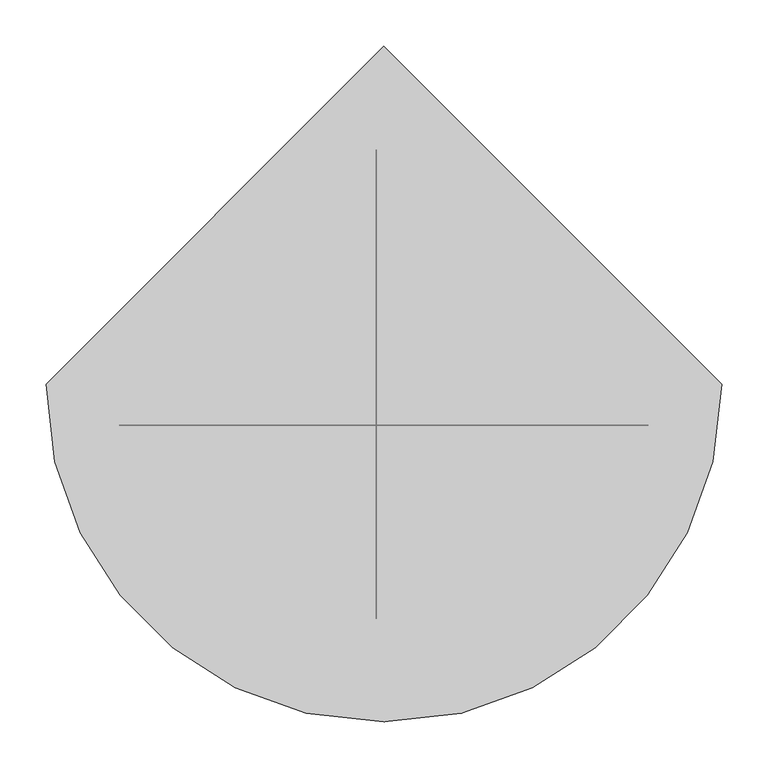
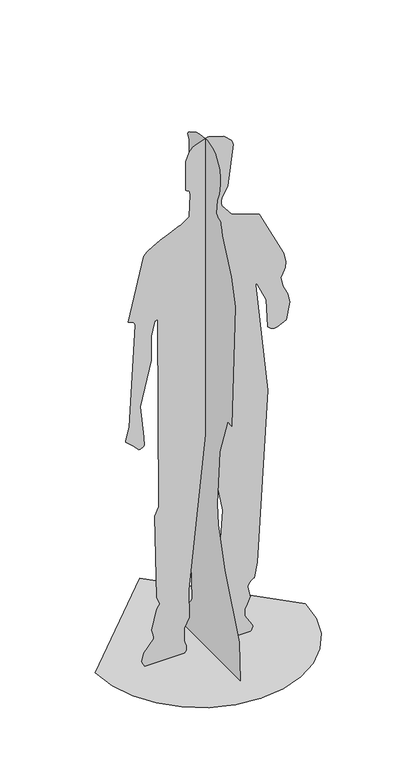
"""IFC4 building model written with IfcOpenShell, lengths in millimetres: proxy geometry, adam 24238 : adam 24238."""

from ifc_helpers import new_model, si_unit, origin, place, context, project, spatial, triangles, source, transform, mapped, element, save


def entourage_3dd67646(model_context):
    return source(origin(), model_context, "Body", "Tessellation", [
        triangles([(-366.6435362, 0.0, 0.0002608), (-356.9509229, -84.0106697, 0.0002608), (-329.3462125, -161.1608025, 0.0002608), (-286.0392629, -229.2406041, 0.0002608), (-229.2406041, -286.0392629, 0.0002608), (-161.1608025, -329.3462125, 0.0002608), (-84.0104153, -356.9509229, 0.0002608), (1.6e-05, -366.6435362, 0.0002608), (84.0106697, -356.9509229, 0.0002608), (161.1608025, -329.3462125, 0.0002608), (229.2406041, -286.0392629, 0.0002608), (286.0392629, -229.2406041, 0.0002608), (329.3462125, -161.1608025, 0.0002608), (356.9509229, -84.0104153, 0.0002608), (366.6435362, 3.21e-05, 0.0002608), (-4.81e-05, 366.6435362, 0.0002608), (-1.944876, -44.4273482, 1879.2018654), (3.9408568, -44.4273482, 1879.5980621), (56.9254043, -44.4273482, 1862.3235352), (60.0092186, -44.4273482, 1860.464201), (82.4127567, -44.4273482, 1839.6871262), (84.7807989, -44.4273482, 1835.3868073), (86.2341804, -44.4273482, 1831.4396645), (87.2151253, -44.4273482, 1827.7541336), (88.1663572, -44.4273482, 1824.2387959), (89.5305907, -44.4273482, 1820.8022324), (69.8819309, -44.4273482, 1675.5804279), (49.8977401, -44.4273482, 1635.9869144), (47.4702674, -44.4273482, 1627.3306114), (46.8911467, -44.4273482, 1618.12565), (48.8728526, -44.4273482, 1608.5092312), (84.8181331, -44.4273482, 1564.6994053), (180.6730562, -44.4273482, 1530.7014805), (265.4856119, -44.4273482, 1357.9816452), (273.9031577, -44.4273482, 1321.9899467), (272.1200725, -44.4273482, 1302.5614815), (259.6918704, -44.4273482, 1276.1125145), (255.5592919, -44.4273482, 1271.5937496), (262.6230323, -44.4273482, 1237.7838947), (280.4588985, -44.4273482, 1201.9495995), (287.0120778, -44.4273482, 1169.7501114), (275.2163406, -44.4273482, 1107.5938036), (243.3053342, -44.4273482, 1092.5062071), (232.2253601, -44.4273482, 1091.4673897), (221.1288717, -44.4273482, 1094.7134851), (210.6275142, -44.4273482, 1103.8498461), (204.6366735, -44.4273482, 1205.693557), (173.7175396, -44.4273482, 1274.9364235), (170.1887216, -44.4273482, 1279.8310375), (168.2918534, -44.4273482, 1273.0009312), (210.6275142, -44.4273482, 870.2031338), (173.1843963, -44.4273482, 247.1475961), (162.7002979, -44.4273482, 193.2292847), (158.5405409, -44.4273482, 191.6712584), (154.4254941, -44.4273482, 189.1513178), (150.5182108, -44.4273482, 185.873193), (143.9807646, -44.4273482, 177.8600194), (140.2342727, -44.4273482, 169.2656857), (139.8659722, -44.4273482, 165.4886996), (148.7468164, -44.4273482, 128.2548804), (146.2251135, -44.4273482, 121.3384694), (135.4476463, -44.4273482, 98.5313222), (129.7501834, -44.4273482, 91.3837752), (130.189855, -44.4273482, 64.5309176), (156.6515392, -44.4273482, 21.8279259), (157.9146888, -44.4273482, 16.6136911), (151.2215381, -44.4273482, 0.0003058), (84.0693416, -44.4273482, 0.0003058), (74.1432851, -44.4273482, 0.0003058), (38.7179401, -44.4273482, 0.0003058), (33.3654053, -44.4273482, 7.4764826), (29.9579983, -44.4273482, 15.6459779), (30.9000852, -44.4273482, 79.4020938), (5.8130383, -44.4273482, 108.6077512), (16.2900951, -44.4273482, 154.9116381), (26.428926, -44.4273482, 174.7358278), (31.8360723, -44.4273482, 178.7200504), (53.3658514, -44.4273482, 480.7935817), (-0.5087539, -44.4273482, 768.3289015), (-4.8489568, -44.4273482, 778.4024872), (-8.1273059, -44.4273482, 782.5858801), (-66.7455444, -44.4273482, 230.3825947), (-64.9545927, -44.4273482, 127.3293101), (-82.1785686, -44.4273482, 92.8816126), (-82.0467452, -44.4273482, 50.1072885), (-79.3850799, -44.4273482, 38.292748), (-77.114579, -44.4273482, 31.7072965), (-75.2644421, -44.4273482, 24.8938543), (-74.7376438, -44.4273482, 21.6405237), (-73.9411035, -44.4273482, 8.9179564), (-82.2286019, -44.4273482, 0.0003058), (-167.3571176, -44.4273482, 0.0003058), (-195.4322207, -44.4273482, 0.0003058), (-220.693524, -44.4273482, 0.0003058), (-229.0292798, -44.4273482, 16.7492252), (-230.8413058, -44.4273482, 20.814543), (-222.9200778, -44.4273482, 48.8121459), (-189.2661364, -44.4273482, 91.3837752), (-188.5071711, -44.4273482, 95.7134528), (-189.5673716, -44.4273482, 106.4002369), (-195.2572133, -44.4273482, 124.3338897), (-177.4482894, -44.4273482, 196.2374042), (-171.6923907, -44.4273482, 207.2632755), (-166.6131586, -44.4273482, 211.9511071), (-178.7820379, -44.4273482, 241.1567554), (-184.9603309, -44.4273482, 542.7618922), (-171.2933599, -44.4273482, 573.6533206), (-173.5918024, -44.4273482, 1268.7160183), (-176.5392242, -44.4273482, 1266.3157288), (-180.7269047, -44.4273482, 1264.2963753), (-184.1635227, -44.4273482, 1262.873933), (-196.7547963, -44.4273482, 1211.6854151), (-197.4888539, -44.4273482, 1123.6948557), (-235.7404617, -44.4273482, 964.4218014), (-222.7747923, -44.4273482, 847.8637997), (-222.2916823, -44.4273482, 817.8105469), (-224.3125073, -44.4273482, 813.6982979), (-236.1842028, -44.4273482, 807.6734476), (-240.250488, -44.4273482, 807.7775837), (-258.0789783, -44.4273482, 826.659934), (-286.6183881, -44.4273482, 852.2301029), (-287.0120778, -44.4273482, 857.7164686), (-274.6372154, -44.4273482, 903.1544655), (-252.8453043, -44.4273482, 1272.1043289), (-256.6642027, -44.4273482, 1280.580265), (-259.0238515, -44.4273482, 1283.9636341), (-262.7017702, -44.4273482, 1287.1919254), (-277.6318727, -44.4273482, 1292.5639812), (-223.7140882, -44.4273482, 1517.22178), (-211.4377663, -44.4273482, 1529.2765675), (-191.0382847, -44.4273482, 1542.4388454), (-166.1168408, -44.4273482, 1555.6290287), (-140.2749134, -44.4273482, 1567.7650612), (-117.1134366, -44.4273482, 1577.7727352), (-100.2331261, -44.4273482, 1584.5672333), (-93.235688, -44.4273482, 1587.0715862), (-64.9545927, -44.4273482, 1608.5092312), (-60.4615893, -44.4273482, 1689.3852539), (-64.9545927, -44.4273482, 1704.3637001), (-72.9002105, -44.4273482, 1706.6725708), (-76.9365194, -44.4273482, 1710.3554855), (-76.9365194, -44.4273482, 1815.1964699), (-63.7389465, -44.4273482, 1845.7348675), (-52.4684725, -44.4273482, 1859.6082939), (-45.3999133, -44.4273482, 1864.0863636), (-8.0256042, -11.9576731, 1872.7679558), (-8.0256042, 11.9818279, 1866.0065952), (-8.0256042, 15.3371645, 1863.8221355), (-8.0256042, 22.6286333, 1860.1111702), (-8.0256042, 52.1745951, 1843.9237862), (-8.0256042, 59.2657593, 1838.2062572), (-8.0256042, 62.1903128, 1832.0620102), (-8.0256042, 53.0188886, 1813.7892883), (-8.0256042, 52.9246538, 1765.8900318), (-8.0256042, 44.5975276, 1745.3719528), (-8.0256042, 43.1614143, 1739.042252), (-8.0256042, 42.5904236, 1733.5252922), (-8.0256042, 43.7575489, 1727.7036999), (-8.0256042, 55.0026293, 1710.038063), (-8.0256042, 56.3198681, 1705.2323971), (-8.0256042, 56.3130144, 1700.5637867), (-8.0256042, 54.9551303, 1697.4193565), (-8.0256042, 51.5324831, 1692.3012096), (-8.0256042, 42.342519, 1638.3515957), (-8.0256042, 37.5670701, 1634.3867214), (-8.0256042, 32.4891075, 1633.1116539), (-8.0256042, 26.9745186, 1632.7509201), (-8.0256042, 10.5312862, 1632.4512291), (-8.0256042, 5.990914, 1631.0491344), (-8.0256042, -10.8585396, 1605.5881886), (-8.0256042, -12.7524636, 1593.756934), (-8.0256042, -14.0942421, 1561.7504574), (-8.0256042, -12.4802009, 1555.913459), (-8.0256042, -0.6249435, 1547.4248783), (-8.0256042, 1.123296, 1487.2675037), (-8.0256042, 62.9045588, 1181.7312841), (-8.0256042, 204.7502021, 1194.7106518), (-8.0256042, 240.9944469, 1187.0627174), (-8.0256042, 245.2555422, 1184.3373024), (-8.0256042, 248.1186306, 1181.6397926), (-8.0256042, 250.7140027, 1178.419059), (-8.0256042, 252.8133113, 1174.7919548), (-8.0256042, 254.190244, 1170.8651596), (-8.0256042, 254.6144186, 1166.7529106), (-8.0256042, 252.0965127, 1160.1615978), (-8.0256042, 209.0618576, 1117.5633259), (-8.0256042, 200.8416653, 1117.1137167), (-8.0256042, 154.1989273, 1133.9615255), (-8.0256042, 137.6038465, 1140.5426645), (-8.0256042, 128.3780742, 1142.4908014), (-8.0256042, 118.7530076, 1142.7423122), (-8.0256042, 91.266931, 1137.6775051), (-8.0256042, 83.8282953, 1135.5007484), (-8.0256042, 77.8819104, 1133.8040497), (-8.0256042, 107.8363502, 921.1249529), (-8.0256042, 77.8819104, 924.1221537), (-8.0256042, 65.8999792, 456.8286927), (-8.0256042, 47.1936582, 374.7740719), (-8.0256042, 36.3199306, 128.765169), (-8.0256042, 38.6638419, 122.1693053), (-8.0256042, 45.3846753, 111.9155889), (-8.0256042, 54.7316111, 99.4668029), (-8.0256042, 64.9538296, 86.2865028), (-8.0256042, 74.3007655, 73.8377259), (-8.0256042, 77.1531849, 69.6548554), (-8.0256042, 85.0581621, 63.3091807), (-8.0256042, 97.368766, 60.2769303), (-8.0256042, 127.5726364, 57.0927906), (-8.0256042, 134.7956331, 56.8740993), (-8.0256042, 155.3528358, 55.5908928), (-8.0256042, 161.7546616, 53.878679), (-8.0256042, 166.2479011, 4.4535808), (-8.0256042, 137.0691771, 0.0002528), (-8.0256042, 128.8367944, 0.0002532), (-8.0256042, 121.8759366, 0.0002535), (-8.0256042, 117.0100635, 0.0002537), (-8.0256042, 48.9467671, 0.0002567), (-8.0256042, 31.4243401, 0.0002575), (-8.0256042, 24.3088155, 0.0002578), (-8.0256042, 0.7015143, 0.0002588), (-8.0256042, -24.0727244, 0.0002599), (-8.0255537, -254.6144186, 0.0), (-8.0255537, -248.6230692, 138.153504), (-8.0256042, -160.756939, 352.2239948), (-8.0256042, -121.7822104, 495.2512384), (-8.0256042, -116.8228656, 570.6561198), (-8.0256042, -131.8002127, 771.3540075), (-8.0256042, -179.7276742, 912.1384375), (-8.0255537, -203.6912733, 909.1437801), (-8.0255537, -226.1570532, 1364.4536339), (-8.0255537, -199.9978759, 1460.4934113), (-8.0256042, -169.3555966, 1535.006741), (-8.0256042, -147.61906, 1580.8308334), (-8.0256042, -142.8377657, 1595.5425808), (-8.0256042, -138.9363323, 1616.7312584), (-8.0256042, -137.2446932, 1621.2904278), (-8.0256042, -133.7301003, 1625.7405922), (-8.0256042, -128.0097736, 1628.0545498), (-8.0256042, -123.0057277, 1629.601403), (-8.0256042, -118.2638024, 1630.7520596), (-8.0256042, -115.801271, 1634.0717697), (-8.0256042, -113.8274453, 1638.5065281), (-8.0256042, -111.5132515, 1642.3217022), (-8.0256042, -117.9460529, 1693.2055149), (-8.0256042, -128.7237653, 1721.4399834), (-8.0256042, -135.6343355, 1760.7313351), (-8.0256042, -135.6241799, 1785.6739986), (-8.0256042, -131.8002127, 1813.7715569), (-8.0256042, -114.0471539, 1843.6088345), (-8.0256042, -105.9849461, 1853.79673), (-8.0256042, -97.1990998, 1861.6657265), (-8.0256042, -86.7393912, 1867.8404949), (-8.0256042, -56.9985558, 1877.6016724)], [[15, 16, 1], [14, 15, 1], [14, 1, 2], [13, 14, 2], [13, 2, 3], [13, 3, 4], [12, 13, 4], [11, 12, 4], [11, 4, 5], [11, 5, 6], [11, 6, 7], [11, 7, 8], [11, 8, 9], [11, 9, 10], [66, 67, 68], [115, 116, 117], [52, 53, 54], [66, 68, 69], [66, 69, 70], [66, 70, 71], [65, 66, 71], [65, 71, 72], [65, 72, 73], [64, 65, 73], [63, 64, 73], [89, 90, 91], [127, 128, 129], [62, 63, 73], [61, 62, 73], [61, 73, 74], [61, 74, 75], [61, 75, 76], [61, 76, 77], [60, 61, 77], [59, 60, 77], [58, 59, 77], [57, 58, 77], [56, 57, 77], [56, 77, 78], [55, 56, 78], [54, 55, 78], [52, 54, 78], [51, 52, 78], [51, 78, 79], [51, 79, 80], [51, 80, 81], [45, 46, 47], [44, 45, 47], [43, 44, 47], [42, 43, 47], [41, 42, 47], [40, 41, 47], [39, 40, 47], [38, 39, 47], [38, 47, 48], [38, 48, 49], [37, 38, 49], [36, 37, 49], [35, 36, 49], [34, 35, 49], [33, 34, 49], [32, 33, 49], [95, 96, 97], [94, 95, 97], [93, 94, 97], [92, 93, 97], [91, 92, 97], [91, 97, 98], [91, 98, 99], [89, 91, 99], [88, 89, 99], [87, 88, 99], [86, 87, 99], [85, 86, 99], [84, 85, 99], [84, 99, 100], [84, 100, 101], [83, 84, 101], [83, 101, 102], [83, 102, 103], [83, 103, 104], [82, 83, 104], [82, 104, 105], [82, 105, 106], [82, 106, 107], [82, 107, 108], [81, 82, 108], [51, 81, 108], [50, 51, 108], [49, 50, 108], [32, 49, 108], [31, 32, 108], [30, 31, 108], [118, 119, 120], [117, 118, 120], [115, 117, 120], [115, 120, 121], [115, 121, 122], [115, 122, 123], [114, 115, 123], [114, 123, 124], [113, 114, 124], [112, 113, 124], [111, 112, 124], [111, 124, 125], [111, 125, 126], [110, 111, 126], [109, 110, 126], [108, 109, 126], [30, 108, 126], [30, 126, 127], [30, 127, 129], [30, 129, 130], [30, 130, 131], [30, 131, 132], [30, 132, 133], [30, 133, 134], [30, 134, 135], [30, 135, 136], [30, 136, 137], [30, 137, 138], [29, 30, 138], [28, 29, 138], [27, 28, 138], [27, 138, 139], [26, 27, 139], [25, 26, 139], [24, 25, 139], [23, 24, 139], [22, 23, 139], [21, 22, 139], [20, 21, 139], [19, 20, 139], [18, 19, 139], [17, 18, 139], [145, 17, 139], [144, 145, 139], [143, 144, 139], [142, 143, 139], [141, 142, 139], [141, 139, 140], [194, 195, 196], [221, 222, 223], [221, 223, 224], [220, 221, 224], [219, 220, 224], [218, 219, 224], [217, 218, 224], [216, 217, 224], [215, 216, 224], [214, 215, 224], [205, 214, 224], [228, 229, 230], [173, 174, 175], [150, 151, 152], [150, 152, 153], [210, 211, 212], [209, 210, 212], [208, 209, 212], [208, 212, 213], [207, 208, 213], [206, 207, 213], [205, 213, 214], [205, 206, 213], [204, 205, 224], [203, 204, 224], [202, 203, 224], [201, 202, 224], [200, 201, 224], [199, 200, 224], [199, 224, 225], [198, 199, 225], [197, 198, 225], [196, 197, 225], [196, 225, 226], [196, 226, 227], [196, 227, 228], [194, 196, 228], [194, 228, 230], [194, 230, 231], [193, 194, 231], [192, 193, 231], [192, 231, 232], [149, 150, 153], [185, 186, 187], [185, 187, 188], [184, 185, 188], [183, 184, 188], [182, 183, 188], [181, 182, 188], [180, 181, 188], [179, 180, 188], [178, 179, 188], [177, 178, 188], [177, 188, 189], [177, 189, 190], [177, 190, 191], [177, 191, 192], [176, 177, 192], [176, 192, 232], [175, 176, 232], [173, 175, 232], [173, 232, 233], [172, 173, 233], [172, 233, 234], [171, 172, 234], [171, 234, 235], [171, 235, 236], [171, 236, 237], [171, 237, 238], [171, 238, 239], [171, 239, 240], [170, 171, 240], [170, 240, 241], [170, 241, 242], [170, 242, 243], [169, 170, 243], [169, 243, 244], [168, 169, 244], [168, 244, 245], [168, 245, 246], [168, 246, 247], [168, 247, 248], [168, 248, 249], [168, 249, 250], [168, 250, 251], [168, 251, 252], [168, 252, 253], [168, 253, 146], [168, 146, 147], [168, 147, 148], [168, 148, 149], [168, 149, 153], [167, 168, 153], [164, 165, 166], [164, 166, 167], [163, 164, 167], [158, 159, 160], [158, 160, 161], [158, 161, 162], [158, 162, 163], [158, 163, 167], [157, 158, 167], [153, 154, 155], [153, 155, 156], [167, 153, 156], [157, 167, 156]], closed=False),
    ])


if __name__ == "__main__":
    model = new_model("IFC4")
    model_context = context("Model", 3, world=origin())
    ifc_project = project(units=[si_unit("LENGTHUNIT", "METRE", prefix="MILLI")], contexts=[model_context])
    site = spatial("IfcSite", under=ifc_project)
    building = spatial("IfcBuilding", under=site)
    placement = place(None, origin())
    entourage_shape = entourage_3dd67646(model_context)
    element("IfcBuildingElementProxy", 1, Name="adam 24238 : adam 24238", ObjectType="adam 24238 : adam 24238", at=placement, inside=building, context=model_context, shape_type="MappedRepresentation", body=[
        mapped(entourage_shape, transform((0.0, 0.0, 0.0), x_axis=(1.0, 0.0, 0.0), y_axis=(0.0, 1.0, 0.0), z_axis=(0.0, 0.0, 1.0))),
    ])
    save(model, "model.ifc")

# Revit data of these elements
# Type "adam 24238 : adam 24238"
#   built-in parameter 1005195 = "RPC-8-G3GT-G6Q0-PL50-C"
#   Height = 0
